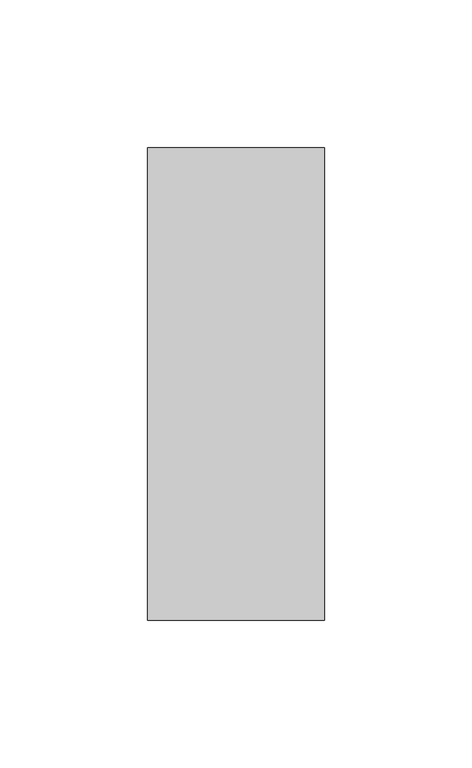
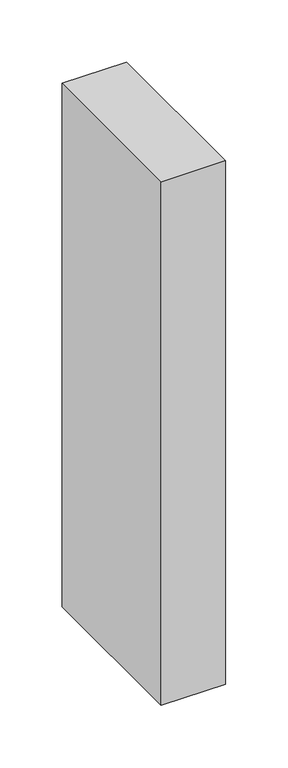
"""IFC4 building model written with IfcOpenShell, lengths in millimetres: column geometry, Madeira de lei-Coluna : Pontalete 6X16cm."""

import ifcopenshell
import ifcopenshell.guid

model = None  # the IFC model being written
_history = None  # IfcOwnerHistory: only IFC2X3 demands one
_inside = {}  # id of a spatial element -> (the spatial element, [elements in it])
_under = {}  # id of a project, library or spatial element -> (it, [spatial elements below it])
_declared = {}  # id of a project -> (the project, [libraries it declares])
_typed = {}  # id of a type object -> (the type object, [elements of that type])
_made_of = {}  # id of a material, layer set ... -> (it, [elements and type objects made of it])


def new_model(schema):
    """Start an empty IFC model of exactly this schema.

    Asked for "IFC4X3", IfcOpenShell would pick the latest addendum, in which some entities
    have other attributes; the version numbers below select the first issue.
    IFC2X3 requires an IfcOwnerHistory on every rooted entity: one is made here for all.
    """
    global model, _history
    if schema == "IFC4X3":
        model = ifcopenshell.file(schema_version=(4, 3, 0, 0))
    else:
        model = ifcopenshell.file(schema=schema)
    _inside.clear()
    _under.clear()
    _declared.clear()
    _typed.clear()
    _made_of.clear()
    _history = None
    if model.schema == "IFC2X3":
        org = make("IfcOrganization", Name="unknown")
        user = make(
            "IfcPersonAndOrganization",
            ThePerson=make("IfcPerson", FamilyName="unknown"),
            TheOrganization=org,
        )
        app = make(
            "IfcApplication",
            ApplicationDeveloper=org,
            Version="unknown",
            ApplicationFullName="unknown",
            ApplicationIdentifier="unknown",
        )
        _history = make(
            "IfcOwnerHistory",
            OwningUser=user,
            OwningApplication=app,
            ChangeAction="ADDED",
            CreationDate=0,
        )
    return model


def make(cls, **values):
    """One entity of the class cls with the attributes given. An attribute that is None is left unset."""
    return model.create_entity(
        cls, **{name: value for name, value in values.items() if value is not None}
    )


def rooted(cls, **values):
    """An entity with a GlobalId (a new one), such as an element, a storey or a relation."""
    return make(cls, GlobalId=ifcopenshell.guid.new(), OwnerHistory=_history, **values)


def si_unit(unit_type, name, prefix=None):
    """IfcSIUnit, for example si_unit("LENGTHUNIT", "METRE", prefix="MILLI")."""
    return make("IfcSIUnit", UnitType=unit_type, Prefix=prefix, Name=name)


def assignment(units):
    """IfcUnitAssignment: the units of a project."""
    return None if units is None else make("IfcUnitAssignment", Units=units)


def point(xyz):
    """IfcCartesianPoint."""
    return None if xyz is None else make("IfcCartesianPoint", Coordinates=xyz)


def direction(xyz):
    """IfcDirection."""
    return None if xyz is None else make("IfcDirection", DirectionRatios=xyz)


def frame(location, z_axis=None, x_axis=None):
    """IfcAxis2Placement3D, a coordinate frame: its origin and axes. An axis left out is left unset."""
    return make(
        "IfcAxis2Placement3D",
        Location=point(location),
        Axis=direction(z_axis),
        RefDirection=direction(x_axis),
    )


def origin():
    """The frame at (0, 0, 0) with its axes left unset."""
    return frame((0.0, 0.0, 0.0))


def place(relative_to, where):
    """IfcLocalPlacement: puts the frame where relative to a parent placement (None: the world)."""
    return make(
        "IfcLocalPlacement", PlacementRelTo=relative_to, RelativePlacement=where
    )


def context(
    kind, dimensions, precision=None, world=None, true_north=None, identifier=None
):
    """IfcGeometricRepresentationContext, for example the 3D "Model" context."""
    return make(
        "IfcGeometricRepresentationContext",
        ContextIdentifier=identifier,
        ContextType=kind,
        CoordinateSpaceDimension=dimensions,
        Precision=precision,
        WorldCoordinateSystem=world,
        TrueNorth=true_north,
    )


def project(units=None, contexts=None):
    """IfcProject with its units and contexts."""
    return rooted(
        "IfcProject",
        Name="project",
        RepresentationContexts=contexts,
        UnitsInContext=assignment(units),
    )


def spatial(cls, under=None, at=None, **own):
    """A site, building, storey or space (cls), placed at a placement, below another one or the project."""
    s = rooted(cls, ObjectPlacement=at, **own)
    if under is not None:
        _under.setdefault(under.id(), (under, []))[1].append(s)
    return s


def polyline(points):
    """IfcPolyline through the points."""
    return make("IfcPolyline", Points=[point(p) for p in points])


def outline(outer, holes=None, kind="AREA"):
    """IfcArbitraryClosedProfileDef: a profile drawn as a closed curve; with holes, ...WithVoids."""
    if holes is None:
        return make("IfcArbitraryClosedProfileDef", ProfileType=kind, OuterCurve=outer)
    return make(
        "IfcArbitraryProfileDefWithVoids",
        ProfileType=kind,
        OuterCurve=outer,
        InnerCurves=holes,
    )


def extrude(swept, where, along, depth):
    """IfcExtrudedAreaSolid: the profile swept, set in the frame where, extruded along a direction by depth."""
    return make(
        "IfcExtrudedAreaSolid",
        SweptArea=swept,
        Position=where,
        ExtrudedDirection=direction(along),
        Depth=depth,
    )


def shape(context_of_items, identifier, shape_type, items):
    """IfcShapeRepresentation: the items that make up one representation, for example the "Body"."""
    return make(
        "IfcShapeRepresentation",
        ContextOfItems=context_of_items,
        RepresentationIdentifier=identifier,
        RepresentationType=shape_type,
        Items=items,
    )


def source(mapping_origin, context_of_items, identifier, shape_type, items):
    """IfcRepresentationMap: a shape defined once, which mapped items show again and again."""
    return make(
        "IfcRepresentationMap",
        MappingOrigin=mapping_origin,
        MappedRepresentation=shape(context_of_items, identifier, shape_type, items),
    )


def transform(
    local_origin,
    x_axis=None,
    y_axis=None,
    z_axis=None,
    scale=None,
    scale2=None,
    scale3=None,
    uniform=True,
):
    """IfcCartesianTransformationOperator3D, or its non-uniform kind. x_axis, y_axis, z_axis: its Axis1, 2, 3."""
    if uniform:
        return make(
            "IfcCartesianTransformationOperator3D",
            Axis1=direction(x_axis),
            Axis2=direction(y_axis),
            LocalOrigin=point(local_origin),
            Scale=scale,
            Axis3=direction(z_axis),
        )
    return make(
        "IfcCartesianTransformationOperator3DnonUniform",
        Axis1=direction(x_axis),
        Axis2=direction(y_axis),
        LocalOrigin=point(local_origin),
        Scale=scale,
        Axis3=direction(z_axis),
        Scale2=scale2,
        Scale3=scale3,
    )


def mapped(mapping_source, mapping_target):
    """IfcMappedItem: shows the shape of a source again, moved by a transform."""
    return make(
        "IfcMappedItem", MappingSource=mapping_source, MappingTarget=mapping_target
    )


def made_of(thing, what):
    """Note that an element or type object is made of a material, layer set ...; save() writes the relation."""
    if what is not None:
        _made_of.setdefault(what.id(), (what, []))[1].append(thing)
    return thing


def element(
    cls,
    number,
    at=None,
    inside=None,
    cuts=None,
    type_object=None,
    material=None,
    context=None,
    identifier="Body",
    shape_type=None,
    held_by="IfcProductDefinitionShape",
    body=None,
    shapes=None,
    **own,
):
    """One element of the class cls, such as IfcWall. Its Tag is "e" and its number.

    at: its placement. inside: the storey or other place that contains it. cuts: it is an
    opening in that element (IfcRelVoidsElement). A single representation is given by context,
    identifier, shape_type and body (its items); several are given by shapes. held_by: the class
    of the entity that holds the representations. save() writes the other relations.
    """
    e = rooted(cls, Tag="e%d" % number, ObjectPlacement=at, **own)
    if body is not None:
        shapes = [shape(context, identifier, shape_type, body)]
    if shapes is not None:
        e.Representation = make(held_by, Representations=shapes)
    if inside is not None:
        _inside.setdefault(inside.id(), (inside, []))[1].append(e)
    if cuts is not None:
        rooted(
            "IfcRelVoidsElement", RelatingBuildingElement=cuts, RelatedOpeningElement=e
        )
    if type_object is not None:
        _typed.setdefault(type_object.id(), (type_object, []))[1].append(e)
    return made_of(e, material)


def aggregate(whole, parts):
    """IfcRelAggregates: a whole, such as a stair, and the parts it consists of."""
    return rooted("IfcRelAggregates", RelatingObject=whole, RelatedObjects=parts)


def save(model, path):
    """Write the relations noted so far, then the file.

    IfcRelAggregates (storeys below a building ...), IfcRelContainedInSpatialStructure (elements
    in a storey), IfcRelDefinesByType, IfcRelAssociatesMaterial and IfcRelDeclares: one each for
    every whole, place, type object, material and project.
    """
    for whole, parts in _under.values():
        aggregate(whole, parts)
    for where, things in _inside.values():
        rooted(
            "IfcRelContainedInSpatialStructure",
            RelatedElements=things,
            RelatingStructure=where,
        )
    for kind, things in _typed.values():
        rooted("IfcRelDefinesByType", RelatedObjects=things, RelatingType=kind)
    for what, things in _made_of.values():
        rooted("IfcRelAssociatesMaterial", RelatedObjects=things, RelatingMaterial=what)
    for by, libraries in _declared.values():
        rooted("IfcRelDeclares", RelatingContext=by, RelatedDefinitions=libraries)
    model.write(path)


def column_e8b88e91(model_context):
    return source(origin(), model_context, "Body", "SweptSolid", [
        extrude(outline(polyline([(30.0, 80.0), (30.0, -80.0), (-30.0, -80.0), (-30.0, 80.0), (30.0, 80.0)])), frame((0.0, 0.0, 6710.0), z_axis=(0.0, 0.0, 1.0), x_axis=(1.0, 0.0, 0.0)), (0.0, 0.0, 1.0), 515.0),
    ])


if __name__ == "__main__":
    model = new_model("IFC4")
    model_context = context("Model", 3, world=origin())
    ifc_project = project(units=[si_unit("LENGTHUNIT", "METRE", prefix="MILLI")], contexts=[model_context])
    site = spatial("IfcSite", under=ifc_project)
    building = spatial("IfcBuilding", under=site)
    placement = place(None, origin())
    column_shape = column_e8b88e91(model_context)
    element("IfcColumn", 1, ObjectType="Madeira de lei-Coluna : Pontalete 6X16cm", at=placement, inside=building, context=model_context, shape_type="MappedRepresentation", body=[
        mapped(column_shape, transform((0.0, 0.0, 0.0), x_axis=(1.0, 0.0, 0.0), y_axis=(0.0, 1.0, 0.0), z_axis=(0.0, 0.0, 1.0))),
    ])
    save(model, "model.ifc")

# Revit data of these elements
# Type "Madeira de lei-Coluna : Pontalete 6X16cm"
#   A = 0.01952 m²
#   b = 0.06 m
#   d = 0.16 m
#   Structural Material [instance default] = none
#   Assembly Code = ""
# Element 1 (IfcColumn, "Madeira de lei-Coluna : Pontalete 6X16cm")
#   Structural Material = .MADEIRAMENTO
#   Materials on its faces: ".MADEIRAMENTO"
# Materials
#   ".MADEIRAMENTO": class ".CC_MADEIRAS", colour RGB 212 179 113, transparency 0, Cost = 0
